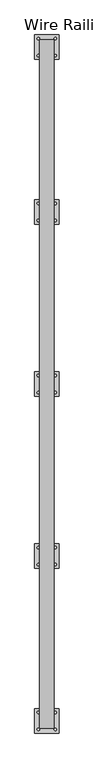
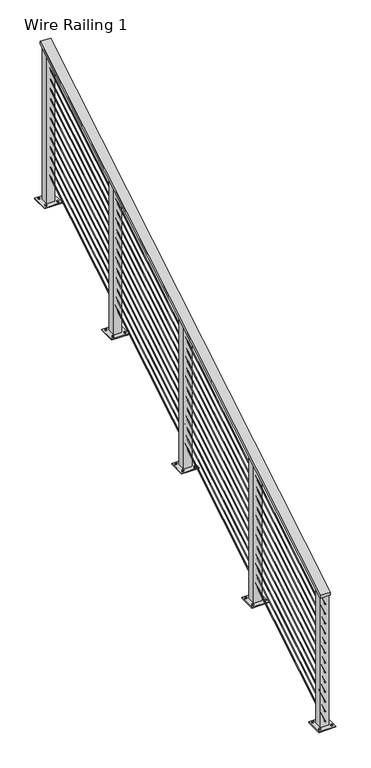
"""IFC4 building model written with IfcOpenShell, lengths in millimetres: railing geometry, Wire Railing 1."""

from ifc_helpers import new_model, si_unit, point, frame, frame_2d, origin, place, context, project, spatial, polyline, circle_curve, ellipse_curve, trimmed, segment, composite_curve, outline, extrude, faceted_brep, source, transform, mapped, element, save
from ifc_brep_helpers import plane_surface, cylinder_surface, advanced_brep


def wire_railing_1_55012836(model_context):
    return source(origin(), model_context, "Body", "SolidModel", [
        faceted_brep([(33186.6840778, 30205.3668167, 267494.1523303), (33186.6840778, 30205.3668167, 267471.9206644), (33262.8840778, 30205.3668167, 267471.9206644), (33262.8840778, 30205.3668167, 267494.1523303), (33186.6840778, 33786.7668167, 269648.7378918), (33262.8840778, 33786.7668167, 269648.7378918), (33262.8840778, 33786.7668167, 269626.5062259), (33186.6840778, 33786.7668167, 269626.5062259)], [[[0, 1, 2, 3]], [[4, 5, 6, 7]], [[1, 0, 4, 7]], [[2, 1, 7, 6]], [[3, 2, 6, 5]], [[0, 3, 5, 4]]]),
        advanced_brep(
        [(33227.1653278, 30205.3668167, 267413.5825391), (33222.4028278, 30205.3668167, 267413.5825391), (33227.1653278, 33786.7668167, 269568.1681006), (33222.4028278, 33786.7668167, 269568.1681006)],
        [
            (0, 1, ellipse_curve(frame((33224.7840778, 30205.3668167, 267413.5825391), z_axis=(0.0, -1.0, 0.0), x_axis=(0.0, 0.0, -1.0)), 2.7789582, 2.38125)),
            (1, 0, ellipse_curve(frame((33224.7840778, 30205.3668167, 267413.5825391), z_axis=(0.0, -1.0, 0.0), x_axis=(0.0, 0.0, -1.0)), 2.7789582, 2.38125)),
            (2, 3, ellipse_curve(frame((33224.7840778, 33786.7668167, 269568.1681006), z_axis=(0.0, 1.0, 0.0), x_axis=(0.0, 0.0, -1.0)), 2.7789582, 2.38125)),
            (3, 2, ellipse_curve(frame((33224.7840778, 33786.7668167, 269568.1681006), z_axis=(0.0, 1.0, 0.0), x_axis=(0.0, 0.0, -1.0)), 2.7789582, 2.38125)),
            (0, 2),
            (3, 1),
        ],
        [
            plane_surface(frame((33224.7840778, 30205.3668167, 267416.3614973), z_axis=(0.0, -1.0, 0.0), x_axis=(0.0, 0.0, 1.0))),
            plane_surface(frame((33224.7840778, 33786.7668167, 269570.9470588), z_axis=(0.0, 1.0, 0.0), x_axis=(0.0, 0.0, 1.0))),
            cylinder_surface(frame((33224.7840778, 30206.5943658, 267414.3210379), z_axis=(0.0, -0.8568858520826494, -0.5155061944347438), x_axis=(-1.0, 0.0, 0.0)), 2.38125),
        ],
        [
            (0, [[1, 2]]),
            (1, [[3, 4]]),
            (2, [[-1, 5, -4, 6]]),
            (2, [[-2, -6, -3, -5]]),
        ],
    ),
        advanced_brep(
        [(33227.1653278, 30205.3668167, 267337.3825391), (33222.4028278, 30205.3668167, 267337.3825391), (33227.1653278, 33786.7668167, 269491.9681006), (33222.4028278, 33786.7668167, 269491.9681006)],
        [
            (0, 1, ellipse_curve(frame((33224.7840778, 30205.3668167, 267337.3825391), z_axis=(0.0, -1.0, 0.0), x_axis=(0.0, 0.0, -1.0)), 2.7789582, 2.38125)),
            (1, 0, ellipse_curve(frame((33224.7840778, 30205.3668167, 267337.3825391), z_axis=(0.0, -1.0, 0.0), x_axis=(0.0, 0.0, -1.0)), 2.7789582, 2.38125)),
            (2, 3, ellipse_curve(frame((33224.7840778, 33786.7668167, 269491.9681006), z_axis=(0.0, 1.0, 0.0), x_axis=(0.0, 0.0, -1.0)), 2.7789582, 2.38125)),
            (3, 2, ellipse_curve(frame((33224.7840778, 33786.7668167, 269491.9681006), z_axis=(0.0, 1.0, 0.0), x_axis=(0.0, 0.0, -1.0)), 2.7789582, 2.38125)),
            (0, 2),
            (3, 1),
        ],
        [
            plane_surface(frame((33224.7840778, 30205.3668167, 267340.1614973), z_axis=(0.0, -1.0, 0.0), x_axis=(0.0, 0.0, 1.0))),
            plane_surface(frame((33224.7840778, 33786.7668167, 269494.7470588), z_axis=(0.0, 1.0, 0.0), x_axis=(0.0, 0.0, 1.0))),
            cylinder_surface(frame((33224.7840778, 30206.5943658, 267338.1210379), z_axis=(0.0, -0.8568858520826494, -0.5155061944347438), x_axis=(-1.0, 0.0, 0.0)), 2.38125),
        ],
        [
            (0, [[1, 2]]),
            (1, [[3, 4]]),
            (2, [[-1, 5, -4, 6]]),
            (2, [[-2, -6, -3, -5]]),
        ],
    ),
        advanced_brep(
        [(33227.1653278, 30205.3668167, 267261.1825391), (33222.4028278, 30205.3668167, 267261.1825391), (33227.1653278, 33786.7668167, 269415.7681006), (33222.4028278, 33786.7668167, 269415.7681006)],
        [
            (0, 1, ellipse_curve(frame((33224.7840778, 30205.3668167, 267261.1825391), z_axis=(0.0, -1.0, 0.0), x_axis=(0.0, 0.0, -1.0)), 2.7789582, 2.38125)),
            (1, 0, ellipse_curve(frame((33224.7840778, 30205.3668167, 267261.1825391), z_axis=(0.0, -1.0, 0.0), x_axis=(0.0, 0.0, -1.0)), 2.7789582, 2.38125)),
            (2, 3, ellipse_curve(frame((33224.7840778, 33786.7668167, 269415.7681006), z_axis=(0.0, 1.0, 0.0), x_axis=(0.0, 0.0, -1.0)), 2.7789582, 2.38125)),
            (3, 2, ellipse_curve(frame((33224.7840778, 33786.7668167, 269415.7681006), z_axis=(0.0, 1.0, 0.0), x_axis=(0.0, 0.0, -1.0)), 2.7789582, 2.38125)),
            (0, 2),
            (3, 1),
        ],
        [
            plane_surface(frame((33224.7840778, 30205.3668167, 267263.9614973), z_axis=(0.0, -1.0, 0.0), x_axis=(0.0, 0.0, 1.0))),
            plane_surface(frame((33224.7840778, 33786.7668167, 269418.5470588), z_axis=(0.0, 1.0, 0.0), x_axis=(0.0, 0.0, 1.0))),
            cylinder_surface(frame((33224.7840778, 30206.5943658, 267261.9210379), z_axis=(0.0, -0.8568858520826494, -0.5155061944347438), x_axis=(-1.0, 0.0, 0.0)), 2.38125),
        ],
        [
            (0, [[1, 2]]),
            (1, [[3, 4]]),
            (2, [[-1, 5, -4, 6]]),
            (2, [[-2, -6, -3, -5]]),
        ],
    ),
        advanced_brep(
        [(33227.1653278, 30205.3668167, 267184.9825391), (33222.4028278, 30205.3668167, 267184.9825391), (33227.1653278, 33786.7668167, 269339.5681006), (33222.4028278, 33786.7668167, 269339.5681006)],
        [
            (0, 1, ellipse_curve(frame((33224.7840778, 30205.3668167, 267184.9825391), z_axis=(0.0, -1.0, 0.0), x_axis=(0.0, 0.0, -1.0)), 2.7789582, 2.38125)),
            (1, 0, ellipse_curve(frame((33224.7840778, 30205.3668167, 267184.9825391), z_axis=(0.0, -1.0, 0.0), x_axis=(0.0, 0.0, -1.0)), 2.7789582, 2.38125)),
            (2, 3, ellipse_curve(frame((33224.7840778, 33786.7668167, 269339.5681006), z_axis=(0.0, 1.0, 0.0), x_axis=(0.0, 0.0, -1.0)), 2.7789582, 2.38125)),
            (3, 2, ellipse_curve(frame((33224.7840778, 33786.7668167, 269339.5681006), z_axis=(0.0, 1.0, 0.0), x_axis=(0.0, 0.0, -1.0)), 2.7789582, 2.38125)),
            (0, 2),
            (3, 1),
        ],
        [
            plane_surface(frame((33224.7840778, 30205.3668167, 267187.7614973), z_axis=(0.0, -1.0, 0.0), x_axis=(0.0, 0.0, 1.0))),
            plane_surface(frame((33224.7840778, 33786.7668167, 269342.3470588), z_axis=(0.0, 1.0, 0.0), x_axis=(0.0, 0.0, 1.0))),
            cylinder_surface(frame((33224.7840778, 30206.5943658, 267185.7210379), z_axis=(0.0, -0.8568858520826494, -0.5155061944347438), x_axis=(-1.0, 0.0, 0.0)), 2.38125),
        ],
        [
            (0, [[1, 2]]),
            (1, [[3, 4]]),
            (2, [[-1, 5, -4, 6]]),
            (2, [[-2, -6, -3, -5]]),
        ],
    ),
        advanced_brep(
        [(33227.1653278, 30205.3668167, 267108.7825391), (33222.4028278, 30205.3668167, 267108.7825391), (33227.1653278, 33786.7668167, 269263.3681006), (33222.4028278, 33786.7668167, 269263.3681006)],
        [
            (0, 1, ellipse_curve(frame((33224.7840778, 30205.3668167, 267108.7825391), z_axis=(0.0, -1.0, 0.0), x_axis=(0.0, 0.0, -1.0)), 2.7789582, 2.38125)),
            (1, 0, ellipse_curve(frame((33224.7840778, 30205.3668167, 267108.7825391), z_axis=(0.0, -1.0, 0.0), x_axis=(0.0, 0.0, -1.0)), 2.7789582, 2.38125)),
            (2, 3, ellipse_curve(frame((33224.7840778, 33786.7668167, 269263.3681006), z_axis=(0.0, 1.0, 0.0), x_axis=(0.0, 0.0, -1.0)), 2.7789582, 2.38125)),
            (3, 2, ellipse_curve(frame((33224.7840778, 33786.7668167, 269263.3681006), z_axis=(0.0, 1.0, 0.0), x_axis=(0.0, 0.0, -1.0)), 2.7789582, 2.38125)),
            (0, 2),
            (3, 1),
        ],
        [
            plane_surface(frame((33224.7840778, 30205.3668167, 267111.5614973), z_axis=(0.0, -1.0, 0.0), x_axis=(0.0, 0.0, 1.0))),
            plane_surface(frame((33224.7840778, 33786.7668167, 269266.1470588), z_axis=(0.0, 1.0, 0.0), x_axis=(0.0, 0.0, 1.0))),
            cylinder_surface(frame((33224.7840778, 30206.5943658, 267109.5210379), z_axis=(0.0, -0.8568858520826494, -0.5155061944347438), x_axis=(-1.0, 0.0, 0.0)), 2.38125),
        ],
        [
            (0, [[1, 2]]),
            (1, [[3, 4]]),
            (2, [[-1, 5, -4, 6]]),
            (2, [[-2, -6, -3, -5]]),
        ],
    ),
        advanced_brep(
        [(33227.1653278, 30205.3668167, 267032.5825391), (33222.4028278, 30205.3668167, 267032.5825391), (33227.1653278, 33786.7668167, 269187.1681006), (33222.4028278, 33786.7668167, 269187.1681006)],
        [
            (0, 1, ellipse_curve(frame((33224.7840778, 30205.3668167, 267032.5825391), z_axis=(0.0, -1.0, 0.0), x_axis=(0.0, 0.0, -1.0)), 2.7789582, 2.38125)),
            (1, 0, ellipse_curve(frame((33224.7840778, 30205.3668167, 267032.5825391), z_axis=(0.0, -1.0, 0.0), x_axis=(0.0, 0.0, -1.0)), 2.7789582, 2.38125)),
            (2, 3, ellipse_curve(frame((33224.7840778, 33786.7668167, 269187.1681006), z_axis=(0.0, 1.0, 0.0), x_axis=(0.0, 0.0, -1.0)), 2.7789582, 2.38125)),
            (3, 2, ellipse_curve(frame((33224.7840778, 33786.7668167, 269187.1681006), z_axis=(0.0, 1.0, 0.0), x_axis=(0.0, 0.0, -1.0)), 2.7789582, 2.38125)),
            (0, 2),
            (3, 1),
        ],
        [
            plane_surface(frame((33224.7840778, 30205.3668167, 267035.3614973), z_axis=(0.0, -1.0, 0.0), x_axis=(0.0, 0.0, 1.0))),
            plane_surface(frame((33224.7840778, 33786.7668167, 269189.9470588), z_axis=(0.0, 1.0, 0.0), x_axis=(0.0, 0.0, 1.0))),
            cylinder_surface(frame((33224.7840778, 30206.5943658, 267033.3210379), z_axis=(0.0, -0.8568858520826494, -0.5155061944347438), x_axis=(-1.0, 0.0, 0.0)), 2.38125),
        ],
        [
            (0, [[1, 2]]),
            (1, [[3, 4]]),
            (2, [[-1, 5, -4, 6]]),
            (2, [[-2, -6, -3, -5]]),
        ],
    ),
        advanced_brep(
        [(33227.1653278, 30205.3668167, 266956.3825391), (33222.4028278, 30205.3668167, 266956.3825391), (33227.1653278, 33786.7668167, 269110.9681006), (33222.4028278, 33786.7668167, 269110.9681006)],
        [
            (0, 1, ellipse_curve(frame((33224.7840778, 30205.3668167, 266956.3825391), z_axis=(0.0, -1.0, 0.0), x_axis=(0.0, 0.0, -1.0)), 2.7789582, 2.38125)),
            (1, 0, ellipse_curve(frame((33224.7840778, 30205.3668167, 266956.3825391), z_axis=(0.0, -1.0, 0.0), x_axis=(0.0, 0.0, -1.0)), 2.7789582, 2.38125)),
            (2, 3, ellipse_curve(frame((33224.7840778, 33786.7668167, 269110.9681006), z_axis=(0.0, 1.0, 0.0), x_axis=(0.0, 0.0, -1.0)), 2.7789582, 2.38125)),
            (3, 2, ellipse_curve(frame((33224.7840778, 33786.7668167, 269110.9681006), z_axis=(0.0, 1.0, 0.0), x_axis=(0.0, 0.0, -1.0)), 2.7789582, 2.38125)),
            (0, 2),
            (3, 1),
        ],
        [
            plane_surface(frame((33224.7840778, 30205.3668167, 266959.1614973), z_axis=(0.0, -1.0, 0.0), x_axis=(0.0, 0.0, 1.0))),
            plane_surface(frame((33224.7840778, 33786.7668167, 269113.7470588), z_axis=(0.0, 1.0, 0.0), x_axis=(0.0, 0.0, 1.0))),
            cylinder_surface(frame((33224.7840778, 30206.5943658, 266957.1210379), z_axis=(0.0, -0.8568858520826494, -0.5155061944347438), x_axis=(-1.0, 0.0, 0.0)), 2.38125),
        ],
        [
            (0, [[1, 2]]),
            (1, [[3, 4]]),
            (2, [[-1, 5, -4, 6]]),
            (2, [[-2, -6, -3, -5]]),
        ],
    ),
        advanced_brep(
        [(33227.1653278, 30205.3668167, 266880.1825391), (33222.4028278, 30205.3668167, 266880.1825391), (33227.1653278, 33786.7668167, 269034.7681006), (33222.4028278, 33786.7668167, 269034.7681006)],
        [
            (0, 1, ellipse_curve(frame((33224.7840778, 30205.3668167, 266880.1825391), z_axis=(0.0, -1.0, 0.0), x_axis=(0.0, 0.0, -1.0)), 2.7789582, 2.38125)),
            (1, 0, ellipse_curve(frame((33224.7840778, 30205.3668167, 266880.1825391), z_axis=(0.0, -1.0, 0.0), x_axis=(0.0, 0.0, -1.0)), 2.7789582, 2.38125)),
            (2, 3, ellipse_curve(frame((33224.7840778, 33786.7668167, 269034.7681006), z_axis=(0.0, 1.0, 0.0), x_axis=(0.0, 0.0, -1.0)), 2.7789582, 2.38125)),
            (3, 2, ellipse_curve(frame((33224.7840778, 33786.7668167, 269034.7681006), z_axis=(0.0, 1.0, 0.0), x_axis=(0.0, 0.0, -1.0)), 2.7789582, 2.38125)),
            (0, 2),
            (3, 1),
        ],
        [
            plane_surface(frame((33224.7840778, 30205.3668167, 266882.9614973), z_axis=(0.0, -1.0, 0.0), x_axis=(0.0, 0.0, 1.0))),
            plane_surface(frame((33224.7840778, 33786.7668167, 269037.5470588), z_axis=(0.0, 1.0, 0.0), x_axis=(0.0, 0.0, 1.0))),
            cylinder_surface(frame((33224.7840778, 30206.5943658, 266880.9210379), z_axis=(0.0, -0.8568858520826494, -0.5155061944347438), x_axis=(-1.0, 0.0, 0.0)), 2.38125),
        ],
        [
            (0, [[1, 2]]),
            (1, [[3, 4]]),
            (2, [[-1, 5, -4, 6]]),
            (2, [[-2, -6, -3, -5]]),
        ],
    ),
        advanced_brep(
        [(33227.1653278, 30205.3668167, 266803.9825391), (33222.4028278, 30205.3668167, 266803.9825391), (33227.1653278, 33786.7668167, 268958.5681006), (33222.4028278, 33786.7668167, 268958.5681006)],
        [
            (0, 1, ellipse_curve(frame((33224.7840778, 30205.3668167, 266803.9825391), z_axis=(0.0, -1.0, 0.0), x_axis=(0.0, 0.0, -1.0)), 2.7789582, 2.38125)),
            (1, 0, ellipse_curve(frame((33224.7840778, 30205.3668167, 266803.9825391), z_axis=(0.0, -1.0, 0.0), x_axis=(0.0, 0.0, -1.0)), 2.7789582, 2.38125)),
            (2, 3, ellipse_curve(frame((33224.7840778, 33786.7668167, 268958.5681006), z_axis=(0.0, 1.0, 0.0), x_axis=(0.0, 0.0, -1.0)), 2.7789582, 2.38125)),
            (3, 2, ellipse_curve(frame((33224.7840778, 33786.7668167, 268958.5681006), z_axis=(0.0, 1.0, 0.0), x_axis=(0.0, 0.0, -1.0)), 2.7789582, 2.38125)),
            (0, 2),
            (3, 1),
        ],
        [
            plane_surface(frame((33224.7840778, 30205.3668167, 266806.7614973), z_axis=(0.0, -1.0, 0.0), x_axis=(0.0, 0.0, 1.0))),
            plane_surface(frame((33224.7840778, 33786.7668167, 268961.3470588), z_axis=(0.0, 1.0, 0.0), x_axis=(0.0, 0.0, 1.0))),
            cylinder_surface(frame((33224.7840778, 30206.5943658, 266804.7210379), z_axis=(0.0, -0.8568858520826494, -0.5155061944347438), x_axis=(-1.0, 0.0, 0.0)), 2.38125),
        ],
        [
            (0, [[1, 2]]),
            (1, [[3, 4]]),
            (2, [[-1, 5, -4, 6]]),
            (2, [[-2, -6, -3, -5]]),
        ],
    ),
        advanced_brep(
        [(33227.1653278, 30205.3668167, 266727.7825391), (33222.4028278, 30205.3668167, 266727.7825391), (33227.1653278, 33786.7668167, 268882.3681006), (33222.4028278, 33786.7668167, 268882.3681006)],
        [
            (0, 1, ellipse_curve(frame((33224.7840778, 30205.3668167, 266727.7825391), z_axis=(0.0, -1.0, 0.0), x_axis=(0.0, 0.0, -1.0)), 2.7789582, 2.38125)),
            (1, 0, ellipse_curve(frame((33224.7840778, 30205.3668167, 266727.7825391), z_axis=(0.0, -1.0, 0.0), x_axis=(0.0, 0.0, -1.0)), 2.7789582, 2.38125)),
            (2, 3, ellipse_curve(frame((33224.7840778, 33786.7668167, 268882.3681006), z_axis=(0.0, 1.0, 0.0), x_axis=(0.0, 0.0, -1.0)), 2.7789582, 2.38125)),
            (3, 2, ellipse_curve(frame((33224.7840778, 33786.7668167, 268882.3681006), z_axis=(0.0, 1.0, 0.0), x_axis=(0.0, 0.0, -1.0)), 2.7789582, 2.38125)),
            (0, 2),
            (3, 1),
        ],
        [
            plane_surface(frame((33224.7840778, 30205.3668167, 266730.5614973), z_axis=(0.0, -1.0, 0.0), x_axis=(0.0, 0.0, 1.0))),
            plane_surface(frame((33224.7840778, 33786.7668167, 268885.1470588), z_axis=(0.0, 1.0, 0.0), x_axis=(0.0, 0.0, 1.0))),
            cylinder_surface(frame((33224.7840778, 30206.5943658, 266728.5210379), z_axis=(0.0, -0.8568858520826494, -0.5155061944347438), x_axis=(-1.0, 0.0, 0.0)), 2.38125),
        ],
        [
            (0, [[1, 2]]),
            (1, [[3, 4]]),
            (2, [[-1, 5, -4, 6]]),
            (2, [[-2, -6, -3, -5]]),
        ],
    ),
        advanced_brep(
        [(33227.1653278, 30205.3668167, 266651.5825391), (33222.4028278, 30205.3668167, 266651.5825391), (33227.1653278, 33786.7668167, 268806.1681006), (33222.4028278, 33786.7668167, 268806.1681006)],
        [
            (0, 1, ellipse_curve(frame((33224.7840778, 30205.3668167, 266651.5825391), z_axis=(0.0, -1.0, 0.0), x_axis=(0.0, 0.0, -1.0)), 2.7789582, 2.38125)),
            (1, 0, ellipse_curve(frame((33224.7840778, 30205.3668167, 266651.5825391), z_axis=(0.0, -1.0, 0.0), x_axis=(0.0, 0.0, -1.0)), 2.7789582, 2.38125)),
            (2, 3, ellipse_curve(frame((33224.7840778, 33786.7668167, 268806.1681006), z_axis=(0.0, 1.0, 0.0), x_axis=(0.0, 0.0, -1.0)), 2.7789582, 2.38125)),
            (3, 2, ellipse_curve(frame((33224.7840778, 33786.7668167, 268806.1681006), z_axis=(0.0, 1.0, 0.0), x_axis=(0.0, 0.0, -1.0)), 2.7789582, 2.38125)),
            (0, 2),
            (3, 1),
        ],
        [
            plane_surface(frame((33224.7840778, 30205.3668167, 266654.3614973), z_axis=(0.0, -1.0, 0.0), x_axis=(0.0, 0.0, 1.0))),
            plane_surface(frame((33224.7840778, 33786.7668167, 268808.9470588), z_axis=(0.0, 1.0, 0.0), x_axis=(0.0, 0.0, 1.0))),
            cylinder_surface(frame((33224.7840778, 30206.5943658, 266652.3210379), z_axis=(0.0, -0.8568858520826494, -0.5155061944347438), x_axis=(-1.0, 0.0, 0.0)), 2.38125),
        ],
        [
            (0, [[1, 2]]),
            (1, [[3, 4]]),
            (2, [[-1, 5, -4, 6]]),
            (2, [[-2, -6, -3, -5]]),
        ],
    ),
        advanced_brep(
        [(33227.1653278, 30205.3668167, 266575.3825391), (33222.4028278, 30205.3668167, 266575.3825391), (33227.1653278, 33786.7668167, 268729.9681006), (33222.4028278, 33786.7668167, 268729.9681006)],
        [
            (0, 1, ellipse_curve(frame((33224.7840778, 30205.3668167, 266575.3825391), z_axis=(0.0, -1.0, 0.0), x_axis=(0.0, 0.0, -1.0)), 2.7789582, 2.38125)),
            (1, 0, ellipse_curve(frame((33224.7840778, 30205.3668167, 266575.3825391), z_axis=(0.0, -1.0, 0.0), x_axis=(0.0, 0.0, -1.0)), 2.7789582, 2.38125)),
            (2, 3, ellipse_curve(frame((33224.7840778, 33786.7668167, 268729.9681006), z_axis=(0.0, 1.0, 0.0), x_axis=(0.0, 0.0, -1.0)), 2.7789582, 2.38125)),
            (3, 2, ellipse_curve(frame((33224.7840778, 33786.7668167, 268729.9681006), z_axis=(0.0, 1.0, 0.0), x_axis=(0.0, 0.0, -1.0)), 2.7789582, 2.38125)),
            (0, 2),
            (3, 1),
        ],
        [
            plane_surface(frame((33224.7840778, 30205.3668167, 266578.1614973), z_axis=(0.0, -1.0, 0.0), x_axis=(0.0, 0.0, 1.0))),
            plane_surface(frame((33224.7840778, 33786.7668167, 268732.7470588), z_axis=(0.0, 1.0, 0.0), x_axis=(0.0, 0.0, 1.0))),
            cylinder_surface(frame((33224.7840778, 30206.5943658, 266576.1210379), z_axis=(0.0, -0.8568858520826494, -0.5155061944347438), x_axis=(-1.0, 0.0, 0.0)), 2.38125),
        ],
        [
            (0, [[1, 2]]),
            (1, [[3, 4]]),
            (2, [[-1, 5, -4, 6]]),
            (2, [[-2, -6, -3, -5]]),
        ],
    ),
        advanced_brep(
        [(33227.1653278, 30205.3668167, 266499.1825391), (33222.4028278, 30205.3668167, 266499.1825391), (33227.1653278, 33786.7668167, 268653.7681006), (33222.4028278, 33786.7668167, 268653.7681006)],
        [
            (0, 1, ellipse_curve(frame((33224.7840778, 30205.3668167, 266499.1825391), z_axis=(0.0, -1.0, 0.0), x_axis=(0.0, 0.0, -1.0)), 2.7789582, 2.38125)),
            (1, 0, ellipse_curve(frame((33224.7840778, 30205.3668167, 266499.1825391), z_axis=(0.0, -1.0, 0.0), x_axis=(0.0, 0.0, -1.0)), 2.7789582, 2.38125)),
            (2, 3, ellipse_curve(frame((33224.7840778, 33786.7668167, 268653.7681006), z_axis=(0.0, 1.0, 0.0), x_axis=(0.0, 0.0, -1.0)), 2.7789582, 2.38125)),
            (3, 2, ellipse_curve(frame((33224.7840778, 33786.7668167, 268653.7681006), z_axis=(0.0, 1.0, 0.0), x_axis=(0.0, 0.0, -1.0)), 2.7789582, 2.38125)),
            (0, 2),
            (3, 1),
        ],
        [
            plane_surface(frame((33224.7840778, 30205.3668167, 266501.9614973), z_axis=(0.0, -1.0, 0.0), x_axis=(0.0, 0.0, 1.0))),
            plane_surface(frame((33224.7840778, 33786.7668167, 268656.5470588), z_axis=(0.0, 1.0, 0.0), x_axis=(0.0, 0.0, 1.0))),
            cylinder_surface(frame((33224.7840778, 30206.5943658, 266499.9210379), z_axis=(0.0, -0.8568858520826494, -0.5155061944347438), x_axis=(-1.0, 0.0, 0.0)), 2.38125),
        ],
        [
            (0, [[1, 2]]),
            (1, [[3, 4]]),
            (2, [[-1, 5, -4, 6]]),
            (2, [[-2, -6, -3, -5]]),
        ],
    ),
        extrude(outline(composite_curve([segment(trimmed(circle_curve(frame_2d((33180.3340778, 32846.9668167)), 6.35), [point((33173.9840778, 32846.9668167))], [point((33186.6840778, 32846.9668167))], False, "CARTESIAN"), True, "CONTINUOUS"), segment(trimmed(circle_curve(frame_2d((33180.3340778, 32846.9668167)), 6.35), [point((33186.6840778, 32846.9668167))], [point((33173.9840778, 32846.9668167))], False, "CARTESIAN"), True, "CONTINUOUS")], self_intersect=False)), frame((0.0, 0.0, 267907.9941176), z_axis=(0.0, 0.0, 1.0), x_axis=(1.0, 0.0, 0.0)), (0.0, 0.0, 1.0), 12.7),
        extrude(outline(composite_curve([segment(trimmed(circle_curve(frame_2d((33269.2340778, 32846.9668167)), 6.35), [point((33262.8840778, 32846.9668167))], [point((33275.5840778, 32846.9668167))], False, "CARTESIAN"), True, "CONTINUOUS"), segment(trimmed(circle_curve(frame_2d((33269.2340778, 32846.9668167)), 6.35), [point((33275.5840778, 32846.9668167))], [point((33262.8840778, 32846.9668167))], False, "CARTESIAN"), True, "CONTINUOUS")], self_intersect=False)), frame((0.0, 0.0, 267907.9941176), z_axis=(0.0, 0.0, 1.0), x_axis=(1.0, 0.0, 0.0)), (0.0, 0.0, 1.0), 12.7),
        extrude(outline(composite_curve([segment(trimmed(circle_curve(frame_2d((33180.3340778, 32935.8668167)), 6.35), [point((33173.9840778, 32935.8668167))], [point((33186.6840778, 32935.8668167))], False, "CARTESIAN"), True, "CONTINUOUS"), segment(trimmed(circle_curve(frame_2d((33180.3340778, 32935.8668167)), 6.35), [point((33186.6840778, 32935.8668167))], [point((33173.9840778, 32935.8668167))], False, "CARTESIAN"), True, "CONTINUOUS")], self_intersect=False)), frame((0.0, 0.0, 267907.9941176), z_axis=(0.0, 0.0, 1.0), x_axis=(1.0, 0.0, 0.0)), (0.0, 0.0, 1.0), 12.7),
        extrude(outline(composite_curve([segment(trimmed(circle_curve(frame_2d((33269.2340778, 32935.8668167)), 6.35), [point((33262.8840778, 32935.8668167))], [point((33275.5840778, 32935.8668167))], False, "CARTESIAN"), True, "CONTINUOUS"), segment(trimmed(circle_curve(frame_2d((33269.2340778, 32935.8668167)), 6.35), [point((33275.5840778, 32935.8668167))], [point((33262.8840778, 32935.8668167))], False, "CARTESIAN"), True, "CONTINUOUS")], self_intersect=False)), frame((0.0, 0.0, 267907.9941176), z_axis=(0.0, 0.0, 1.0), x_axis=(1.0, 0.0, 0.0)), (0.0, 0.0, 1.0), 12.7),
        extrude(outline(polyline([(33288.2840778, 32827.9168167), (33161.2840778, 32827.9168167), (33161.2840778, 32954.9168167), (33288.2840778, 32954.9168167), (33288.2840778, 32827.9168167)])), frame((0.0, 0.0, 267907.9941176), z_axis=(0.0, 0.0, 1.0), x_axis=(1.0, 0.0, 0.0)), (0.0, 0.0, 1.0), 6.35),
        extrude(outline(polyline([(33254.9465778, 32861.2543167), (33194.6215778, 32861.2543167), (33194.6215778, 32921.5793167), (33254.9465778, 32921.5793167), (33254.9465778, 32861.2543167)]), holes=[polyline([(33248.5965778, 32867.6043167), (33248.5965778, 32915.2293167), (33200.9715778, 32915.2293167), (33200.9715778, 32867.6043167), (33248.5965778, 32867.6043167)])]), frame((0.0, 0.0, 267907.9941176), z_axis=(0.0, 0.0, 1.0), x_axis=(1.0, 0.0, 0.0)), (0.0, 0.0, 1.0), 1179.8657178),
        extrude(outline(composite_curve([segment(trimmed(circle_curve(frame_2d((33180.3340778, 31951.6168167)), 6.35), [point((33173.9840778, 31951.6168167))], [point((33186.6840778, 31951.6168167))], False, "CARTESIAN"), True, "CONTINUOUS"), segment(trimmed(circle_curve(frame_2d((33180.3340778, 31951.6168167)), 6.35), [point((33186.6840778, 31951.6168167))], [point((33173.9840778, 31951.6168167))], False, "CARTESIAN"), True, "CONTINUOUS")], self_intersect=False)), frame((0.0, 0.0, 267403.7294118), z_axis=(0.0, 0.0, 1.0), x_axis=(1.0, 0.0, 0.0)), (0.0, 0.0, 1.0), 12.7),
        extrude(outline(composite_curve([segment(trimmed(circle_curve(frame_2d((33269.2340778, 31951.6168167)), 6.35), [point((33262.8840778, 31951.6168167))], [point((33275.5840778, 31951.6168167))], False, "CARTESIAN"), True, "CONTINUOUS"), segment(trimmed(circle_curve(frame_2d((33269.2340778, 31951.6168167)), 6.35), [point((33275.5840778, 31951.6168167))], [point((33262.8840778, 31951.6168167))], False, "CARTESIAN"), True, "CONTINUOUS")], self_intersect=False)), frame((0.0, 0.0, 267403.7294118), z_axis=(0.0, 0.0, 1.0), x_axis=(1.0, 0.0, 0.0)), (0.0, 0.0, 1.0), 12.7),
        extrude(outline(composite_curve([segment(trimmed(circle_curve(frame_2d((33180.3340778, 32040.5168167)), 6.35), [point((33173.9840778, 32040.5168167))], [point((33186.6840778, 32040.5168167))], False, "CARTESIAN"), True, "CONTINUOUS"), segment(trimmed(circle_curve(frame_2d((33180.3340778, 32040.5168167)), 6.35), [point((33186.6840778, 32040.5168167))], [point((33173.9840778, 32040.5168167))], False, "CARTESIAN"), True, "CONTINUOUS")], self_intersect=False)), frame((0.0, 0.0, 267403.7294118), z_axis=(0.0, 0.0, 1.0), x_axis=(1.0, 0.0, 0.0)), (0.0, 0.0, 1.0), 12.7),
        extrude(outline(composite_curve([segment(trimmed(circle_curve(frame_2d((33269.2340778, 32040.5168167)), 6.35), [point((33262.8840778, 32040.5168167))], [point((33275.5840778, 32040.5168167))], False, "CARTESIAN"), True, "CONTINUOUS"), segment(trimmed(circle_curve(frame_2d((33269.2340778, 32040.5168167)), 6.35), [point((33275.5840778, 32040.5168167))], [point((33262.8840778, 32040.5168167))], False, "CARTESIAN"), True, "CONTINUOUS")], self_intersect=False)), frame((0.0, 0.0, 267403.7294118), z_axis=(0.0, 0.0, 1.0), x_axis=(1.0, 0.0, 0.0)), (0.0, 0.0, 1.0), 12.7),
        extrude(outline(polyline([(33288.2840778, 31932.5668167), (33161.2840778, 31932.5668167), (33161.2840778, 32059.5668167), (33288.2840778, 32059.5668167), (33288.2840778, 31932.5668167)])), frame((0.0, 0.0, 267403.7294118), z_axis=(0.0, 0.0, 1.0), x_axis=(1.0, 0.0, 0.0)), (0.0, 0.0, 1.0), 6.35),
        extrude(outline(polyline([(33254.9465778, 31965.9043167), (33194.6215778, 31965.9043167), (33194.6215778, 32026.2293167), (33254.9465778, 32026.2293167), (33254.9465778, 31965.9043167)]), holes=[polyline([(33248.5965778, 31972.2543167), (33248.5965778, 32019.8793167), (33200.9715778, 32019.8793167), (33200.9715778, 31972.2543167), (33248.5965778, 31972.2543167)])]), frame((0.0, 0.0, 267403.7294118), z_axis=(0.0, 0.0, 1.0), x_axis=(1.0, 0.0, 0.0)), (0.0, 0.0, 1.0), 1145.4840333),
        extrude(outline(composite_curve([segment(trimmed(circle_curve(frame_2d((33180.3340778, 31056.2668167)), 6.35), [point((33173.9840778, 31056.2668167))], [point((33186.6840778, 31056.2668167))], False, "CARTESIAN"), True, "CONTINUOUS"), segment(trimmed(circle_curve(frame_2d((33180.3340778, 31056.2668167)), 6.35), [point((33186.6840778, 31056.2668167))], [point((33173.9840778, 31056.2668167))], False, "CARTESIAN"), True, "CONTINUOUS")], self_intersect=False)), frame((0.0, 0.0, 266899.4647059), z_axis=(0.0, 0.0, 1.0), x_axis=(1.0, 0.0, 0.0)), (0.0, 0.0, 1.0), 12.7),
        extrude(outline(composite_curve([segment(trimmed(circle_curve(frame_2d((33269.2340778, 31056.2668167)), 6.35), [point((33262.8840778, 31056.2668167))], [point((33275.5840778, 31056.2668167))], False, "CARTESIAN"), True, "CONTINUOUS"), segment(trimmed(circle_curve(frame_2d((33269.2340778, 31056.2668167)), 6.35), [point((33275.5840778, 31056.2668167))], [point((33262.8840778, 31056.2668167))], False, "CARTESIAN"), True, "CONTINUOUS")], self_intersect=False)), frame((0.0, 0.0, 266899.4647059), z_axis=(0.0, 0.0, 1.0), x_axis=(1.0, 0.0, 0.0)), (0.0, 0.0, 1.0), 12.7),
        extrude(outline(composite_curve([segment(trimmed(circle_curve(frame_2d((33180.3340778, 31145.1668167)), 6.35), [point((33173.9840778, 31145.1668167))], [point((33186.6840778, 31145.1668167))], False, "CARTESIAN"), True, "CONTINUOUS"), segment(trimmed(circle_curve(frame_2d((33180.3340778, 31145.1668167)), 6.35), [point((33186.6840778, 31145.1668167))], [point((33173.9840778, 31145.1668167))], False, "CARTESIAN"), True, "CONTINUOUS")], self_intersect=False)), frame((0.0, 0.0, 266899.4647059), z_axis=(0.0, 0.0, 1.0), x_axis=(1.0, 0.0, 0.0)), (0.0, 0.0, 1.0), 12.7),
        extrude(outline(composite_curve([segment(trimmed(circle_curve(frame_2d((33269.2340778, 31145.1668167)), 6.35), [point((33262.8840778, 31145.1668167))], [point((33275.5840778, 31145.1668167))], False, "CARTESIAN"), True, "CONTINUOUS"), segment(trimmed(circle_curve(frame_2d((33269.2340778, 31145.1668167)), 6.35), [point((33275.5840778, 31145.1668167))], [point((33262.8840778, 31145.1668167))], False, "CARTESIAN"), True, "CONTINUOUS")], self_intersect=False)), frame((0.0, 0.0, 266899.4647059), z_axis=(0.0, 0.0, 1.0), x_axis=(1.0, 0.0, 0.0)), (0.0, 0.0, 1.0), 12.7),
        extrude(outline(polyline([(33288.2840778, 31037.2168167), (33161.2840778, 31037.2168167), (33161.2840778, 31164.2168167), (33288.2840778, 31164.2168167), (33288.2840778, 31037.2168167)])), frame((0.0, 0.0, 266899.4647059), z_axis=(0.0, 0.0, 1.0), x_axis=(1.0, 0.0, 0.0)), (0.0, 0.0, 1.0), 6.35),
        extrude(outline(polyline([(33254.9465778, 31070.5543167), (33194.6215778, 31070.5543167), (33194.6215778, 31130.8793167), (33254.9465778, 31130.8793167), (33254.9465778, 31070.5543167)]), holes=[polyline([(33248.5965778, 31076.9043167), (33248.5965778, 31124.5293167), (33200.9715778, 31124.5293167), (33200.9715778, 31076.9043167), (33248.5965778, 31076.9043167)])]), frame((0.0, 0.0, 266899.4647059), z_axis=(0.0, 0.0, 1.0), x_axis=(1.0, 0.0, 0.0)), (0.0, 0.0, 1.0), 1111.1023489),
        extrude(outline(composite_curve([segment(trimmed(circle_curve(frame_2d((33180.3340778, 33704.2168167)), 6.35), [point((33173.9840778, 33704.2168167))], [point((33186.6840778, 33704.2168167))], False, "CARTESIAN"), True, "CONTINUOUS"), segment(trimmed(circle_curve(frame_2d((33180.3340778, 33704.2168167)), 6.35), [point((33186.6840778, 33704.2168167))], [point((33173.9840778, 33704.2168167))], False, "CARTESIAN"), True, "CONTINUOUS")], self_intersect=False)), frame((0.0, 0.0, 268412.2588235), z_axis=(0.0, 0.0, 1.0), x_axis=(1.0, 0.0, 0.0)), (0.0, 0.0, 1.0), 12.7),
        extrude(outline(composite_curve([segment(trimmed(circle_curve(frame_2d((33269.2340778, 33704.2168167)), 6.35), [point((33262.8840778, 33704.2168167))], [point((33275.5840778, 33704.2168167))], False, "CARTESIAN"), True, "CONTINUOUS"), segment(trimmed(circle_curve(frame_2d((33269.2340778, 33704.2168167)), 6.35), [point((33275.5840778, 33704.2168167))], [point((33262.8840778, 33704.2168167))], False, "CARTESIAN"), True, "CONTINUOUS")], self_intersect=False)), frame((0.0, 0.0, 268412.2588235), z_axis=(0.0, 0.0, 1.0), x_axis=(1.0, 0.0, 0.0)), (0.0, 0.0, 1.0), 12.7),
        extrude(outline(composite_curve([segment(trimmed(circle_curve(frame_2d((33180.3340778, 33793.1168167)), 6.35), [point((33173.9840778, 33793.1168167))], [point((33186.6840778, 33793.1168167))], False, "CARTESIAN"), True, "CONTINUOUS"), segment(trimmed(circle_curve(frame_2d((33180.3340778, 33793.1168167)), 6.35), [point((33186.6840778, 33793.1168167))], [point((33173.9840778, 33793.1168167))], False, "CARTESIAN"), True, "CONTINUOUS")], self_intersect=False)), frame((0.0, 0.0, 268412.2588235), z_axis=(0.0, 0.0, 1.0), x_axis=(1.0, 0.0, 0.0)), (0.0, 0.0, 1.0), 12.7),
        extrude(outline(composite_curve([segment(trimmed(circle_curve(frame_2d((33269.2340778, 33793.1168167)), 6.35), [point((33262.8840778, 33793.1168167))], [point((33275.5840778, 33793.1168167))], False, "CARTESIAN"), True, "CONTINUOUS"), segment(trimmed(circle_curve(frame_2d((33269.2340778, 33793.1168167)), 6.35), [point((33275.5840778, 33793.1168167))], [point((33262.8840778, 33793.1168167))], False, "CARTESIAN"), True, "CONTINUOUS")], self_intersect=False)), frame((0.0, 0.0, 268412.2588235), z_axis=(0.0, 0.0, 1.0), x_axis=(1.0, 0.0, 0.0)), (0.0, 0.0, 1.0), 12.7),
        extrude(outline(polyline([(33288.2840778, 33685.1668167), (33161.2840778, 33685.1668167), (33161.2840778, 33812.1668167), (33288.2840778, 33812.1668167), (33288.2840778, 33685.1668167)])), frame((0.0, 0.0, 268412.2588235), z_axis=(0.0, 0.0, 1.0), x_axis=(1.0, 0.0, 0.0)), (0.0, 0.0, 1.0), 6.35),
        extrude(outline(polyline([(33254.9465778, 33718.5043167), (33194.6215778, 33718.5043167), (33194.6215778, 33778.8293167), (33254.9465778, 33778.8293167), (33254.9465778, 33718.5043167)]), holes=[polyline([(33248.5965778, 33724.8543167), (33248.5965778, 33772.4793167), (33200.9715778, 33772.4793167), (33200.9715778, 33724.8543167), (33248.5965778, 33724.8543167)])]), frame((0.0, 0.0, 268412.2588235), z_axis=(0.0, 0.0, 1.0), x_axis=(1.0, 0.0, 0.0)), (0.0, 0.0, 1.0), 1191.3262793),
        extrude(outline(composite_curve([segment(trimmed(circle_curve(frame_2d((33180.3340778, 30199.0168167)), 6.35), [point((33173.9840778, 30199.0168167))], [point((33186.6840778, 30199.0168167))], False, "CARTESIAN"), True, "CONTINUOUS"), segment(trimmed(circle_curve(frame_2d((33180.3340778, 30199.0168167)), 6.35), [point((33186.6840778, 30199.0168167))], [point((33173.9840778, 30199.0168167))], False, "CARTESIAN"), True, "CONTINUOUS")], self_intersect=False)), frame((0.0, 0.0, 266448.6826203), z_axis=(0.0, 0.0, 1.0), x_axis=(1.0, 0.0, 0.0)), (0.0, 0.0, 1.0), 12.7),
        extrude(outline(composite_curve([segment(trimmed(circle_curve(frame_2d((33269.2340778, 30199.0168167)), 6.35), [point((33262.8840778, 30199.0168167))], [point((33275.5840778, 30199.0168167))], False, "CARTESIAN"), True, "CONTINUOUS"), segment(trimmed(circle_curve(frame_2d((33269.2340778, 30199.0168167)), 6.35), [point((33275.5840778, 30199.0168167))], [point((33262.8840778, 30199.0168167))], False, "CARTESIAN"), True, "CONTINUOUS")], self_intersect=False)), frame((0.0, 0.0, 266448.6826203), z_axis=(0.0, 0.0, 1.0), x_axis=(1.0, 0.0, 0.0)), (0.0, 0.0, 1.0), 12.7),
        extrude(outline(composite_curve([segment(trimmed(circle_curve(frame_2d((33180.3340778, 30287.9168167)), 6.35), [point((33173.9840778, 30287.9168167))], [point((33186.6840778, 30287.9168167))], False, "CARTESIAN"), True, "CONTINUOUS"), segment(trimmed(circle_curve(frame_2d((33180.3340778, 30287.9168167)), 6.35), [point((33186.6840778, 30287.9168167))], [point((33173.9840778, 30287.9168167))], False, "CARTESIAN"), True, "CONTINUOUS")], self_intersect=False)), frame((0.0, 0.0, 266448.6826203), z_axis=(0.0, 0.0, 1.0), x_axis=(1.0, 0.0, 0.0)), (0.0, 0.0, 1.0), 12.7),
        extrude(outline(composite_curve([segment(trimmed(circle_curve(frame_2d((33269.2340778, 30287.9168167)), 6.35), [point((33262.8840778, 30287.9168167))], [point((33275.5840778, 30287.9168167))], False, "CARTESIAN"), True, "CONTINUOUS"), segment(trimmed(circle_curve(frame_2d((33269.2340778, 30287.9168167)), 6.35), [point((33275.5840778, 30287.9168167))], [point((33262.8840778, 30287.9168167))], False, "CARTESIAN"), True, "CONTINUOUS")], self_intersect=False)), frame((0.0, 0.0, 266448.6826203), z_axis=(0.0, 0.0, 1.0), x_axis=(1.0, 0.0, 0.0)), (0.0, 0.0, 1.0), 12.7),
        extrude(outline(polyline([(33288.2840778, 30179.9668167), (33161.2840778, 30179.9668167), (33161.2840778, 30306.9668167), (33288.2840778, 30306.9668167), (33288.2840778, 30179.9668167)])), frame((0.0, 0.0, 266448.6826203), z_axis=(0.0, 0.0, 1.0), x_axis=(1.0, 0.0, 0.0)), (0.0, 0.0, 1.0), 6.35),
        extrude(outline(polyline([(33254.9465778, 30213.3043167), (33194.6215778, 30213.3043167), (33194.6215778, 30273.6293167), (33254.9465778, 30273.6293167), (33254.9465778, 30213.3043167)]), holes=[polyline([(33248.5965778, 30219.6543167), (33248.5965778, 30267.2793167), (33200.9715778, 30267.2793167), (33200.9715778, 30219.6543167), (33248.5965778, 30219.6543167)])]), frame((0.0, 0.0, 266448.6826203), z_axis=(0.0, 0.0, 1.0), x_axis=(1.0, 0.0, 0.0)), (0.0, 0.0, 1.0), 1046.159167),
    ])


if __name__ == "__main__":
    model = new_model("IFC4")
    model_context = context("Model", 3, world=origin())
    ifc_project = project(units=[si_unit("LENGTHUNIT", "METRE", prefix="MILLI")], contexts=[model_context])
    site = spatial("IfcSite", under=ifc_project)
    building = spatial("IfcBuilding", under=site)
    placement = place(None, origin())
    wire_railing_1_shape = wire_railing_1_55012836(model_context)
    element("IfcRailing", 1, ObjectType="Wire Railing 1", at=placement, inside=building, context=model_context, shape_type="MappedRepresentation", body=[
        mapped(wire_railing_1_shape, transform((0.0, 0.0, 0.0), x_axis=(1.0, 0.0, 0.0), y_axis=(0.0, 1.0, 0.0), z_axis=(0.0, 0.0, 1.0))),
    ])
    save(model, "model.ifc")

# Revit data of these elements
# Element 1 (IfcRailing, "Wire Railing 1")
#   Materials on its faces: "2 1/2\" X 2 1/2\" ALUM. SQUARE POST (38\" O.C. MAX)", "WIRE RAILING (3\" O.C.)", "ALUM. PLATE TOP RAIL"
# Materials
#   "2 1/2\" X 2 1/2\" ALUM. SQUARE POST (38\" O.C. MAX)": class "Metal", colour RGB 244 244 244, transparency 0, Manufacturer = "Kawneer", URL = "http://www.kawneer.com/kawneer/north_america/en/home.asp", Cost = 0
#   "WIRE RAILING (3\" O.C.)": class "Metal", colour RGB 244 244 244, transparency 0, Manufacturer = "Kawneer", URL = "http://www.kawneer.com/kawneer/north_america/en/home.asp", Cost = 0
#   "ALUM. PLATE TOP RAIL": class "Metal", colour RGB 244 244 244, transparency 0, Manufacturer = "Kawneer", URL = "http://www.kawneer.com/kawneer/north_america/en/home.asp", Cost = 0
